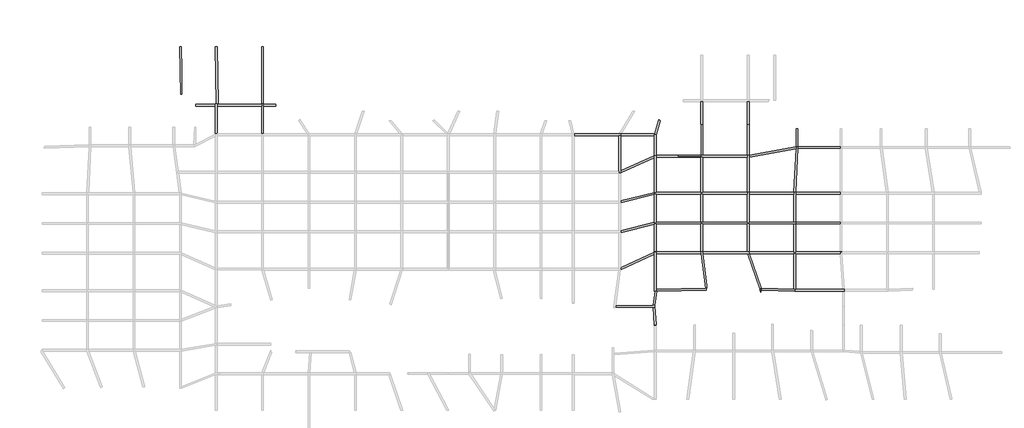
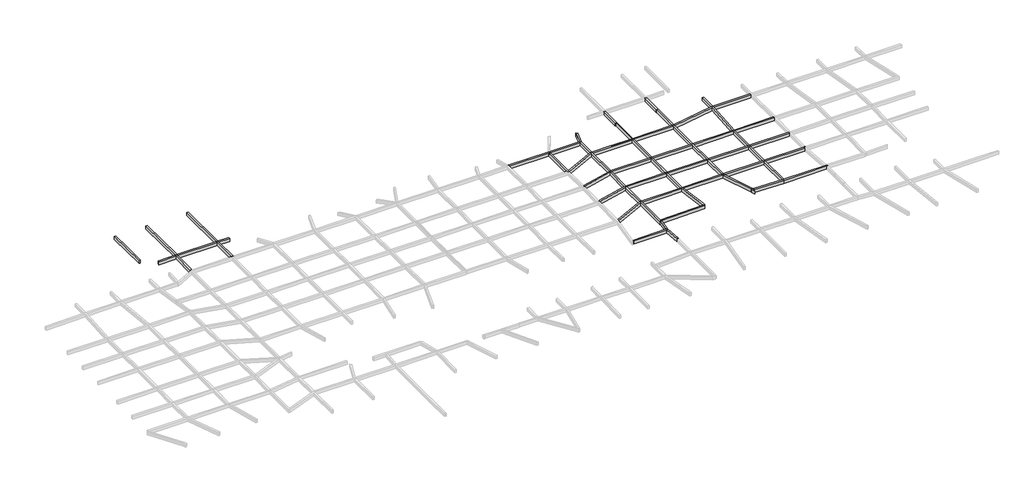
# One storey, part 12 of 15: 57 beams.
"""IFC4 building model written with IfcOpenShell, lengths in millimetres."""

from ifc_helpers import new_model, si_unit, frame, origin, place, context, project, spatial, polyline, outline, extrude, faceted_brep, element, save

model = new_model("IFC4")

# Units and contexts
model_context = context("Model", 3, world=origin())
ifc_project = project(units=[si_unit("LENGTHUNIT", "METRE", prefix="MILLI")], contexts=[model_context])

# Site, building, storey
site = spatial("IfcSite", under=ifc_project)
building = spatial("IfcBuilding", under=site)
storey = spatial("IfcBuildingStorey", under=building, Name="层高", Elevation=3300.0)

# Beams
placement = place(None, origin())
element("IfcBeam", 1, ObjectType="混凝土 - 矩形梁 : KL_beam", at=placement, inside=storey, context=model_context, shape_type="Brep", body=[
    faceted_brep([(161650.3009383, 131842.1448334, 3300.0), (161350.3009383, 131842.1448334, 3300.0), (161350.3009383, 131792.1448334, 3300.0), (161350.3009383, 131492.1448334, 3300.0), (161350.3009383, 126792.1448334, 3300.0), (161650.3009383, 126792.1448334, 3300.0), (161650.3009383, 131492.1448334, 3300.0), (161650.3009383, 131792.1448334, 3300.0), (161650.3009383, 131842.1448334, 2700.0), (161650.3009383, 126792.1448334, 2700.0), (161650.3009383, 131492.1448334, 2700.0), (161650.3009383, 131792.1448334, 2700.0), (161350.3009383, 131842.1448334, 2700.0), (161350.3009383, 126792.1448334, 2700.0), (161350.3009383, 131492.1448334, 2700.0), (161350.3009383, 131792.1448334, 2700.0)], [[[0, 1, 2, 3, 4, 5, 6, 7]], [[8, 0, 7, 6, 5, 9, 10, 11]], [[12, 8, 11, 10, 9, 13, 14, 15]], [[1, 12, 15, 14, 13, 4, 3, 2]], [[5, 4, 13, 9]], [[1, 0, 8, 12]]]),
])
element("IfcBeam", 2, ObjectType="混凝土 - 矩形梁 : KL_beam", at=placement, inside=storey, context=model_context, shape_type="Brep", body=[
    faceted_brep([(221650.3009384, 126492.1448336, 2700.0), (221650.3009384, 126492.1448336, 3300.0), (221350.3009384, 126492.1448336, 3300.0), (213892.2921833, 126492.1448336, 3300.0), (213892.2921833, 126492.1448336, 2700.0), (221350.3009384, 126492.1448336, 2700.0), (213850.3009384, 126792.1448336, 3300.0), (213850.3009384, 126792.1448336, 2700.0), (213850.3009384, 126660.5625177, 2700.0), (213850.3009384, 126660.5625177, 3300.0), (221650.3009384, 126792.1448336, 3300.0), (221414.7215056, 126792.1448336, 3300.0), (221650.3009384, 126792.1448336, 2700.0), (221414.7215056, 126792.1448336, 2700.0)], [[[0, 1, 2, 3, 4, 5]], [[6, 7, 8, 9]], [[1, 10, 11, 6, 9, 3, 2]], [[12, 0, 5, 4, 8, 7, 13]], [[7, 6, 11, 10, 12, 13]], [[4, 3, 9, 8]], [[10, 1, 0, 12]]]),
])
element("IfcBeam", 3, ObjectType="混凝土 - 矩形梁 : KL_beam", at=placement, inside=storey, context=model_context, shape_type="Brep", body=[
    faceted_brep([(221350.3009384, 120192.1448334, 3300.0), (221650.3009384, 120192.1448334, 3300.0), (221650.3009384, 120245.163893, 3300.0), (221650.3009384, 120574.149183, 3300.0), (221650.3009384, 126492.1448336, 3300.0), (221350.3009384, 126492.1448336, 3300.0), (221350.3009384, 120492.1448334, 3300.0), (221650.3009384, 120192.1448334, 2700.0), (221650.3009384, 120245.163893, 2700.0), (221650.3009384, 120574.149183, 2700.0), (221650.3009384, 126492.1448336, 2700.0), (221350.3009384, 120192.1448334, 2700.0), (221350.3009384, 120492.1448334, 2700.0), (221350.3009384, 126492.1448336, 2700.0)], [[[0, 1, 2, 3, 4, 5, 6]], [[1, 7, 8, 9, 10, 4, 3, 2]], [[7, 11, 12, 13, 10, 9, 8]], [[11, 0, 6, 5, 13, 12]], [[5, 4, 10, 13]], [[1, 0, 11, 7]]]),
])
element("IfcBeam", 4, ObjectType="混凝土 - 矩形梁 : KL_beam", at=placement, inside=storey, context=model_context, shape_type="Brep", body=[
    faceted_brep([(227649.8041274, 106937.1819374, 3300.0), (227349.8041274, 106937.1819374, 3300.0), (227349.8041274, 106606.1286193, 3300.0), (227349.8041274, 100394.2440803, 3300.0), (227649.8041274, 100394.2440803, 3300.0), (227649.8041274, 100694.2897788, 3300.0), (227649.8041274, 106691.6486698, 3300.0), (227649.8041274, 106937.1819374, 2700.0), (227649.8041274, 100394.2440803, 2700.0), (227649.8041274, 100694.2897788, 2700.0), (227649.8041274, 106691.6486698, 2700.0), (227349.8041274, 106937.1819374, 2700.0), (227349.8041274, 100394.2440803, 2700.0), (227349.8041274, 106606.1286193, 2700.0)], [[[0, 1, 2, 3, 4, 5, 6]], [[7, 0, 6, 5, 4, 8, 9, 10]], [[11, 7, 10, 9, 8, 12, 13]], [[1, 11, 13, 12, 3, 2]], [[1, 0, 7, 11]], [[3, 12, 8, 4]]]),
])
element("IfcBeam", 5, ObjectType="混凝土 - 矩形梁 : KL_beam", at=placement, inside=storey, context=model_context, shape_type="SweptSolid", body=[
    extrude(outline(polyline([(221650.3009384, 103946.6115658), (221650.3009384, 104032.4006699), (221684.3757671, 104293.5649694), (227349.8041274, 106937.1819374), (227349.8041274, 106606.1286193), (221650.3009384, 103946.6115658)])), frame((0.0, 0.0, 2700.0), z_axis=(0.0, 0.0, 1.0), x_axis=(1.0, 0.0, 0.0)), (0.0, 0.0, 1.0), 600.0),
])
element("IfcBeam", 6, ObjectType="混凝土 - 矩形梁 : KL_beam", at=placement, inside=storey, context=model_context, shape_type="Brep", body=[
    faceted_brep([(227649.8041274, 100694.2897788, 3300.0), (227649.8041274, 100394.2440803, 3300.0), (227761.1939201, 100396.1883964, 3300.0), (236039.6710138, 100540.6897516, 3300.0), (236039.6710138, 100732.444127, 3300.0), (236039.6710138, 100840.73545, 3300.0), (235928.1373023, 100838.7886218, 3300.0), (227349.8041274, 100389.0075609, 3300.0), (227349.8041274, 100389.0075609, 2700.0), (227457.5006433, 100390.8874105, 2700.0), (227649.8041274, 100394.2440803, 2700.0), (227761.1939201, 100396.1883964, 2700.0), (236039.6710138, 100540.6897516, 2700.0), (227457.5006433, 100390.8874105, 3300.0), (227649.8041274, 100694.2897788, 2700.0), (235928.1373023, 100838.7886218, 2700.0), (236039.6710138, 100840.73545, 2700.0), (227349.8041274, 100394.2440803, 3300.0), (227349.8041274, 100394.2440803, 2700.0)], [[[0, 1, 2, 3, 4, 5, 6]], [[7, 8, 9, 10, 11, 12, 3, 2, 1, 13]], [[10, 14, 15, 16, 12, 11]], [[14, 0, 6, 5, 16, 15]], [[8, 7, 17, 18]], [[10, 1, 0, 14]], [[1, 10, 18, 17]], [[17, 7, 13, 1]], [[8, 18, 10, 9]], [[3, 12, 16, 5, 4]]]),
])
element("IfcBeam", 7, ObjectType="混凝土 - 矩形梁 : KL_beam", at=placement, inside=storey, context=model_context, shape_type="Brep", body=[
    faceted_brep([(235431.5832734, 106991.6486698, 3300.0), (235149.8041274, 106991.6486698, 3300.0), (235129.0639103, 106991.6486698, 3300.0), (235168.0249813, 106691.6486698, 3300.0), (235928.1373023, 100838.7886218, 3300.0), (236039.6710138, 100840.73545, 3300.0), (236039.6710138, 100852.444127, 3300.0), (236159.6710138, 100852.444127, 3300.0), (236159.6710138, 101385.3776888, 3300.0), (235470.5443444, 106691.6486698, 3300.0), (235928.1373023, 100838.7886218, 2700.0), (235129.0639103, 106991.6486698, 2700.0), (235168.0249813, 106691.6486698, 2700.0), (235149.8041274, 106991.6486698, 2700.0), (235431.5832734, 106991.6486698, 2700.0), (235470.5443444, 106691.6486698, 2700.0), (236159.6710138, 101385.3776888, 2700.0), (236159.6710138, 100852.444127, 2700.0), (236039.6710138, 100852.444127, 2700.0), (236039.6710138, 100840.73545, 2700.0)], [[[0, 1, 2, 3, 4, 5, 6, 7, 8, 9]], [[10, 4, 3, 2, 11, 12]], [[11, 13, 14, 15, 16, 17, 18, 19, 10, 12]], [[14, 0, 9, 8, 16, 15]], [[4, 10, 19, 5]], [[2, 1, 0, 14, 13, 11]], [[16, 8, 7, 17]], [[6, 18, 17, 7]], [[18, 6, 5, 19]]]),
])
element("IfcBeam", 8, ObjectType="混凝土 - 矩形梁 : KL_beam", at=placement, inside=storey, context=model_context, shape_type="Brep", body=[
    faceted_brep([(227349.8041274, 106991.6486698, 3300.0), (227349.8041274, 106937.1819374, 3300.0), (227649.8041274, 106937.1819374, 3300.0), (227649.8041274, 106746.1154023, 3300.0), (227649.8041274, 106691.6486698, 3300.0), (235168.0249813, 106691.6486698, 3300.0), (235129.0639103, 106991.6486698, 3300.0), (227649.8041274, 106991.6486698, 3300.0), (227649.8041274, 106691.6486698, 2700.0), (235168.0249813, 106691.6486698, 2700.0), (227349.8041274, 106937.1819374, 2700.0), (227349.8041274, 106991.6486698, 2700.0), (227649.8041274, 106991.6486698, 2700.0), (235129.0639103, 106991.6486698, 2700.0), (227649.8041274, 106746.1154023, 2700.0), (227649.8041274, 106937.1819374, 2700.0)], [[[0, 1, 2, 3, 4, 5, 6, 7]], [[4, 8, 9, 5]], [[10, 11, 12, 13, 9, 8, 14, 15]], [[11, 0, 7, 6, 13, 12]], [[0, 11, 10, 1]], [[8, 4, 3, 2, 15, 14]], [[6, 5, 9, 13]], [[15, 2, 1, 10]]]),
])
element("IfcBeam", 9, ObjectType="混凝土 - 矩形梁 : KL_beam", at=placement, inside=storey, context=model_context, shape_type="Brep", body=[
    faceted_brep([(235431.5832734, 106991.6486698, 3300.0), (235470.5443444, 106691.6486698, 3300.0), (242992.8101672, 106691.6486698, 3300.0), (243310.0963715, 106691.6486698, 3300.0), (243249.8041274, 106866.7500612, 3300.0), (243206.7980875, 106991.6486698, 3300.0), (242949.8041274, 106991.6486698, 3300.0), (235449.8041274, 106991.6486698, 3300.0), (235470.5443444, 106691.6486698, 2700.0), (242992.8101672, 106691.6486698, 2700.0), (243310.0963715, 106691.6486698, 2700.0), (235431.5832734, 106991.6486698, 2700.0), (235449.8041274, 106991.6486698, 2700.0), (242949.8041274, 106991.6486698, 2700.0), (243206.7980875, 106991.6486698, 2700.0), (243249.8041274, 106866.7500612, 2700.0)], [[[0, 1, 2, 3, 4, 5, 6, 7]], [[1, 8, 9, 10, 3, 2]], [[8, 11, 12, 13, 14, 15, 10, 9]], [[11, 0, 7, 6, 5, 14, 13, 12]], [[1, 0, 11, 8]], [[5, 4, 3, 10, 15, 14]]]),
])
element("IfcBeam", 10, ObjectType="混凝土 - 矩形梁 : KL_beam", at=placement, inside=storey, context=model_context, shape_type="SweptSolid", body=[
    extrude(outline(polyline([(245239.6710138, 100732.444127), (245239.6710138, 100166.2909583), (245044.7288445, 100732.444127), (245239.6710138, 100732.444127)])), frame((0.0, 0.0, 2700.0), z_axis=(0.0, 0.0, 1.0), x_axis=(1.0, 0.0, 0.0)), (0.0, 0.0, 1.0), 600.0),
    extrude(outline(polyline([(242992.8101672, 106691.6486698), (243310.0963715, 106691.6486698), (245320.6957353, 100852.444127), (245003.4095309, 100852.444127), (242992.8101672, 106691.6486698)])), frame((0.0, 0.0, 2700.0), z_axis=(0.0, 0.0, 1.0), x_axis=(1.0, 0.0, 0.0)), (0.0, 0.0, 1.0), 600.0),
])
element("IfcBeam", 11, ObjectType="混凝土 - 矩形梁 : KL_beam", at=placement, inside=storey, context=model_context, shape_type="Brep", body=[
    faceted_brep([(250897.7707068, 100391.6486698, 3300.0), (250901.8375479, 100691.6486698, 3300.0), (250749.8041274, 100695.7713993, 3300.0), (245359.6710138, 100841.9370275, 3300.0), (245359.6710138, 100541.8267459, 3300.0), (250901.8375479, 100691.6486698, 2700.0), (250749.8041274, 100695.7713993, 2700.0), (245359.6710138, 100841.9370275, 2700.0), (250897.7707068, 100391.6486698, 2700.0), (245359.6710138, 100541.8267459, 2700.0)], [[[0, 1, 2, 3, 4]], [[1, 5, 6, 7, 3, 2]], [[5, 8, 9, 7, 6]], [[8, 0, 4, 9]], [[0, 8, 5, 1]], [[3, 7, 9, 4]]]),
])
element("IfcBeam", 12, ObjectType="混凝土 - 矩形梁 : KL_beam", at=placement, inside=storey, context=model_context, shape_type="Brep", body=[
    faceted_brep([(250901.8375479, 100691.6486698, 3300.0), (250897.7707068, 100391.6486698, 3300.0), (258971.6890495, 100391.6486698, 3300.0), (259271.6890495, 100391.6486698, 3300.0), (259271.6890495, 100546.8867852, 3300.0), (259271.6890495, 100691.6486698, 3300.0), (259261.5663125, 100691.6486698, 3300.0), (258960.833743, 100691.6486698, 3300.0), (251049.8041274, 100691.6486698, 3300.0), (250897.7707068, 100391.6486698, 2700.0), (258971.6890495, 100391.6486698, 2700.0), (259271.6890495, 100391.6486698, 2700.0), (250901.8375479, 100691.6486698, 2700.0), (251049.8041274, 100691.6486698, 2700.0), (258960.833743, 100691.6486698, 2700.0), (259261.5663125, 100691.6486698, 2700.0), (259271.6890495, 100691.6486698, 2700.0), (259271.6890495, 100546.8867852, 2700.0)], [[[0, 1, 2, 3, 4, 5, 6, 7, 8]], [[1, 9, 10, 11, 3, 2]], [[9, 12, 13, 14, 15, 16, 17, 11, 10]], [[12, 0, 8, 7, 6, 5, 16, 15, 14, 13]], [[0, 12, 9, 1]], [[5, 4, 3, 11, 17, 16]]]),
])
element("IfcBeam", 13, ObjectType="混凝土 - 矩形梁 : KL_beam", at=placement, inside=storey, context=model_context, shape_type="Brep", body=[
    faceted_brep([(242949.8041274, 111691.6486698, 3300.0), (243249.8041274, 111691.6486698, 3300.0), (243249.8041274, 111991.6486698, 3300.0), (243249.8041274, 116691.6486698, 3300.0), (243249.8041274, 116991.6486698, 3300.0), (242949.8041274, 116991.6486698, 3300.0), (242949.8041274, 116691.6486698, 3300.0), (242949.8041274, 111991.6486698, 3300.0), (242949.8041274, 111691.6486698, 2700.0), (242949.8041274, 116991.6486698, 2700.0), (242949.8041274, 116691.6486698, 2700.0), (242949.8041274, 111991.6486698, 2700.0), (243249.8041274, 111691.6486698, 2700.0), (243249.8041274, 116991.6486698, 2700.0), (243249.8041274, 116691.6486698, 2700.0), (243249.8041274, 111991.6486698, 2700.0)], [[[0, 1, 2, 3, 4, 5, 6, 7]], [[8, 0, 7, 6, 5, 9, 10, 11]], [[12, 8, 11, 10, 9, 13, 14, 15]], [[1, 12, 15, 14, 13, 4, 3, 2]], [[1, 0, 8, 12]], [[5, 4, 13, 9]]]),
])
element("IfcBeam", 14, ObjectType="混凝土 - 矩形梁 : KL_beam", at=placement, inside=storey, context=model_context, shape_type="Brep", body=[
    faceted_brep([(251049.8041274, 111691.6486698, 3300.0), (251049.8041274, 111991.6486698, 3300.0), (250749.8041274, 111991.6486698, 3300.0), (243249.8041274, 111991.6486698, 3300.0), (243249.8041274, 111691.6486698, 3300.0), (250749.8041274, 111691.6486698, 3300.0), (251049.8041274, 111991.6486698, 2700.0), (250749.8041274, 111991.6486698, 2700.0), (243249.8041274, 111991.6486698, 2700.0), (251049.8041274, 111691.6486698, 2700.0), (250749.8041274, 111691.6486698, 2700.0), (243249.8041274, 111691.6486698, 2700.0)], [[[0, 1, 2, 3, 4, 5]], [[1, 6, 7, 8, 3, 2]], [[6, 9, 10, 11, 8, 7]], [[9, 0, 5, 4, 11, 10]], [[4, 3, 8, 11]], [[1, 0, 9, 6]]]),
])
element("IfcBeam", 15, ObjectType="混凝土 - 矩形梁 : KL_beam", at=placement, inside=storey, context=model_context, shape_type="Brep", body=[
    faceted_brep([(251049.8041274, 116991.6486698, 3300.0), (250757.4594423, 116991.6486698, 3300.0), (250749.8041274, 116991.6486698, 3300.0), (250749.8041274, 116691.6486698, 3300.0), (250749.8041274, 111991.6486698, 3300.0), (251049.8041274, 111991.6486698, 3300.0), (251049.8041274, 116691.6486698, 3300.0), (250749.8041274, 116991.6486698, 2700.0), (250749.8041274, 116691.6486698, 2700.0), (250749.8041274, 111991.6486698, 2700.0), (250757.4594423, 116991.6486698, 2700.0), (251049.8041274, 116991.6486698, 2700.0), (251049.8041274, 116691.6486698, 2700.0), (251049.8041274, 111991.6486698, 2700.0)], [[[0, 1, 2, 3, 4, 5, 6]], [[2, 7, 8, 9, 4, 3]], [[7, 10, 11, 12, 13, 9, 8]], [[11, 0, 6, 5, 13, 12]], [[5, 4, 9, 13]], [[2, 1, 0, 11, 10, 7]]]),
])
element("IfcBeam", 16, ObjectType="混凝土 - 矩形梁 : KL_beam", at=placement, inside=storey, context=model_context, shape_type="SweptSolid", body=[
    extrude(outline(polyline([(243249.8041274, 116691.6486698), (243249.8041274, 116991.6486698), (250749.8041274, 116991.6486698), (250749.8041274, 116691.6486698), (243249.8041274, 116691.6486698)])), frame((0.0, 0.0, 2700.0), z_axis=(0.0, 0.0, 1.0), x_axis=(1.0, 0.0, 0.0)), (0.0, 0.0, 1.0), 600.0),
])
element("IfcBeam", 17, ObjectType="混凝土 - 矩形梁 : KL_beam", at=placement, inside=storey, context=model_context, shape_type="Brep", body=[
    faceted_brep([(235149.8041274, 116991.6486698, 3300.0), (235149.8041274, 116691.6486698, 3300.0), (235449.8041274, 116691.6486698, 3300.0), (242949.8041274, 116691.6486698, 3300.0), (242949.8041274, 116991.6486698, 3300.0), (235449.8041274, 116991.6486698, 3300.0), (235149.8041274, 116691.6486698, 2700.0), (235449.8041274, 116691.6486698, 2700.0), (242949.8041274, 116691.6486698, 2700.0), (235149.8041274, 116991.6486698, 2700.0), (235449.8041274, 116991.6486698, 2700.0), (242949.8041274, 116991.6486698, 2700.0)], [[[0, 1, 2, 3, 4, 5]], [[1, 6, 7, 8, 3, 2]], [[6, 9, 10, 11, 8, 7]], [[9, 0, 5, 4, 11, 10]], [[4, 3, 8, 11]], [[1, 0, 9, 6]]]),
])
element("IfcBeam", 18, ObjectType="混凝土 - 矩形梁 : KL_beam", at=placement, inside=storey, context=model_context, shape_type="Brep", body=[
    faceted_brep([(235149.8041274, 111991.6486698, 3300.0), (235149.8041274, 111691.6486698, 3300.0), (235449.8041274, 111691.6486698, 3300.0), (242949.8041274, 111691.6486698, 3300.0), (242949.8041274, 111991.6486698, 3300.0), (235449.8041274, 111991.6486698, 3300.0), (235149.8041274, 111691.6486698, 2700.0), (235449.8041274, 111691.6486698, 2700.0), (242949.8041274, 111691.6486698, 2700.0), (235149.8041274, 111991.6486698, 2700.0), (235449.8041274, 111991.6486698, 2700.0), (242949.8041274, 111991.6486698, 2700.0)], [[[0, 1, 2, 3, 4, 5]], [[1, 6, 7, 8, 3, 2]], [[6, 9, 10, 11, 8, 7]], [[9, 0, 5, 4, 11, 10]], [[4, 3, 8, 11]], [[1, 0, 9, 6]]]),
])
element("IfcBeam", 19, ObjectType="混凝土 - 矩形梁 : KL_beam", at=placement, inside=storey, context=model_context, shape_type="SweptSolid", body=[
    extrude(outline(polyline([(235149.8041274, 116691.6486698), (235449.8041274, 116691.6486698), (235449.8041274, 111991.6486698), (235149.8041274, 111991.6486698), (235149.8041274, 116691.6486698)])), frame((0.0, 0.0, 2700.0), z_axis=(0.0, 0.0, 1.0), x_axis=(1.0, 0.0, 0.0)), (0.0, 0.0, 1.0), 600.0),
])
element("IfcBeam", 20, ObjectType="混凝土 - 矩形梁 : KL_beam", at=placement, inside=storey, context=model_context, shape_type="Brep", body=[
    faceted_brep([(243249.8041274, 123192.3894162, 3300.0), (242949.8041274, 123192.3894162, 3300.0), (242949.8041274, 122892.3894162, 3300.0), (242949.8041274, 116991.6486698, 3300.0), (243249.8041274, 116991.6486698, 3300.0), (243249.8041274, 122917.161732, 3300.0), (242949.8041274, 123192.3894162, 2700.0), (242949.8041274, 122892.3894162, 2700.0), (242949.8041274, 116991.6486698, 2700.0), (243249.8041274, 123192.3894162, 2700.0), (243249.8041274, 122917.161732, 2700.0), (243249.8041274, 116991.6486698, 2700.0)], [[[0, 1, 2, 3, 4, 5]], [[1, 6, 7, 8, 3, 2]], [[6, 9, 10, 11, 8, 7]], [[9, 0, 5, 4, 11, 10]], [[4, 3, 8, 11]], [[1, 0, 9, 6]]]),
])
element("IfcBeam", 21, ObjectType="混凝土 - 矩形梁 : KL_beam", at=placement, inside=storey, context=model_context, shape_type="Brep", body=[
    faceted_brep([(242949.8041274, 122892.3894162, 3300.0), (242949.8041274, 123192.3894162, 3300.0), (235449.8041274, 123192.3894162, 3300.0), (235209.8041277, 123192.3894162, 3300.0), (235209.8041277, 122892.3894162, 3300.0), (235449.8041274, 122892.3894162, 3300.0), (242949.8041274, 122892.3894162, 2700.0), (235209.8041277, 122892.3894162, 2700.0), (235449.8041274, 122892.3894162, 2700.0), (242949.8041274, 123192.3894162, 2700.0), (235209.8041277, 123192.3894162, 2700.0), (235449.8041274, 123192.3894162, 2700.0)], [[[0, 1, 2, 3, 4, 5]], [[6, 0, 5, 4, 7, 8]], [[9, 6, 8, 7, 10, 11]], [[1, 9, 11, 10, 3, 2]], [[1, 0, 6, 9]], [[4, 3, 10, 7]]]),
])
element("IfcBeam", 22, ObjectType="混凝土 - 矩形梁 : KL_beam", at=placement, inside=storey, context=model_context, shape_type="Brep", body=[
    faceted_brep([(235149.8041274, 116991.6486698, 3300.0), (235449.8041274, 116991.6486698, 3300.0), (235449.8041274, 122892.3894162, 3300.0), (235209.8041277, 122892.3894162, 3300.0), (235149.8041274, 122892.3894162, 3300.0), (235449.8041274, 116991.6486698, 2700.0), (235449.8041274, 122892.3894162, 2700.0), (235149.8041274, 116991.6486698, 2700.0), (235149.8041274, 122892.3894162, 2700.0), (235209.8041277, 122892.3894162, 2700.0)], [[[0, 1, 2, 3, 4]], [[1, 5, 6, 2]], [[5, 7, 8, 9, 6]], [[7, 0, 4, 8]], [[1, 0, 7, 5]], [[4, 3, 2, 6, 9, 8]]]),
])
element("IfcBeam", 23, ObjectType="混凝土 - 矩形梁 : KL_beam", at=placement, inside=storey, context=model_context, shape_type="Brep", body=[
    faceted_brep([(227349.8041274, 116991.6486698, 3300.0), (227349.8041274, 116958.7721753, 3300.0), (227349.8041274, 116691.6486698, 3300.0), (227518.2655284, 116691.6486698, 3300.0), (227649.8041274, 116691.6486698, 3300.0), (235149.8041274, 116691.6486698, 3300.0), (235149.8041274, 116991.6486698, 3300.0), (227649.8041274, 116991.6486698, 3300.0), (227349.8041274, 116691.6486698, 2700.0), (227518.2655284, 116691.6486698, 2700.0), (227649.8041274, 116691.6486698, 2700.0), (235149.8041274, 116691.6486698, 2700.0), (227349.8041274, 116958.7721753, 2700.0), (227349.8041274, 116991.6486698, 2700.0), (227649.8041274, 116991.6486698, 2700.0), (235149.8041274, 116991.6486698, 2700.0)], [[[0, 1, 2, 3, 4, 5, 6, 7]], [[2, 8, 9, 10, 11, 5, 4, 3]], [[8, 12, 13, 14, 15, 11, 10, 9]], [[13, 0, 7, 6, 15, 14]], [[6, 5, 11, 15]], [[2, 1, 0, 13, 12, 8]]]),
])
element("IfcBeam", 24, ObjectType="混凝土 - 矩形梁 : KL_beam", at=placement, inside=storey, context=model_context, shape_type="Brep", body=[
    faceted_brep([(227649.8041274, 123139.3703566, 3300.0), (227349.8041274, 123139.3703566, 3300.0), (227349.8041274, 122810.3850665, 3300.0), (227349.8041274, 116991.6486698, 3300.0), (227649.8041274, 116991.6486698, 3300.0), (227649.8041274, 122892.3894162, 3300.0), (227349.8041274, 123139.3703566, 2700.0), (227349.8041274, 122810.3850665, 2700.0), (227349.8041274, 116991.6486698, 2700.0), (227649.8041274, 123139.3703566, 2700.0), (227649.8041274, 122892.3894162, 2700.0), (227649.8041274, 116991.6486698, 2700.0)], [[[0, 1, 2, 3, 4, 5]], [[1, 6, 7, 8, 3, 2]], [[6, 9, 10, 11, 8, 7]], [[9, 0, 5, 4, 11, 10]], [[4, 3, 8, 11]], [[0, 9, 6, 1]]]),
])
element("IfcBeam", 25, ObjectType="混凝土 - 矩形梁 : KL_beam", at=placement, inside=storey, context=model_context, shape_type="Brep", body=[
    faceted_brep([(227649.8041274, 126621.0726799, 3300.0), (227349.8041274, 126663.2169868, 3300.0), (227349.8041274, 126492.1448336, 3300.0), (227349.8041274, 123139.3703566, 3300.0), (227649.8041274, 123139.3703566, 3300.0), (227649.8041274, 123192.3894162, 3300.0), (227649.8041274, 126621.0726799, 2700.0), (227649.8041274, 123139.3703566, 2700.0), (227649.8041274, 123192.3894162, 2700.0), (227349.8041274, 126663.2169868, 2700.0), (227349.8041274, 123139.3703566, 2700.0), (227349.8041274, 126492.1448336, 2700.0)], [[[0, 1, 2, 3, 4, 5]], [[6, 0, 5, 4, 7, 8]], [[9, 6, 8, 7, 10, 11]], [[1, 9, 11, 10, 3, 2]], [[4, 3, 10, 7]], [[1, 0, 6, 9]]]),
])
element("IfcBeam", 26, ObjectType="混凝土 - 矩形梁 : KL_beam", at=placement, inside=storey, context=model_context, shape_type="Brep", body=[
    faceted_brep([(227349.8041274, 123139.3703566, 3300.0), (221650.3009384, 120574.149183, 3300.0), (221650.3009384, 120492.1448334, 3300.0), (221650.3009384, 120245.163893, 3300.0), (227349.8041274, 122810.3850665, 3300.0), (221650.3009384, 120245.163893, 2700.0), (227349.8041274, 122810.3850665, 2700.0), (221650.3009384, 120574.149183, 2700.0), (227349.8041274, 123139.3703566, 2700.0), (221650.3009384, 120492.1448334, 2700.0)], [[[0, 1, 2, 3, 4]], [[3, 5, 6, 4]], [[7, 8, 6, 5, 9]], [[1, 0, 8, 7]], [[5, 3, 2, 1, 7, 9]], [[0, 4, 6, 8]]]),
])
element("IfcBeam", 27, ObjectType="混凝土 - 矩形梁 : KL_beam", at=placement, inside=storey, context=model_context, shape_type="Brep", body=[
    faceted_brep([(221518.7623395, 115192.1448334, 3300.0), (221350.3009384, 115192.1448334, 3300.0), (221350.3009384, 115150.0399275, 3300.0), (221350.3009384, 115192.1448334, 2700.0), (221518.7623395, 115192.1448334, 2700.0), (221350.3009384, 115150.0399275, 2700.0)], [[[0, 1, 2]], [[3, 4, 5]], [[2, 5, 4, 0]], [[5, 2, 1, 3]], [[1, 0, 4, 3]]]),
    faceted_brep([(221650.3009384, 115534.2497393, 2700.0), (221650.3009384, 115534.2497393, 3300.0), (227349.8041274, 116958.7721753, 3300.0), (227349.8041274, 116958.7721753, 2700.0), (221650.3009384, 115492.1448334, 2700.0), (221650.3009384, 115225.0213279, 2700.0), (221650.3009384, 115225.0213279, 3300.0), (221650.3009384, 115492.1448334, 3300.0), (227349.8041274, 116691.6486698, 2700.0), (227349.8041274, 116691.6486698, 3300.0), (227518.2655284, 116691.6486698, 3300.0), (227518.2655284, 116691.6486698, 2700.0), (227349.8041274, 116649.5437639, 3300.0), (227349.8041274, 116649.5437639, 2700.0)], [[[0, 1, 2, 3]], [[1, 0, 4, 5, 6, 7]], [[8, 9, 10, 11]], [[9, 8, 3, 2]], [[6, 12, 10, 9, 2, 1, 7]], [[0, 3, 8, 11, 13, 5, 4]], [[6, 5, 13, 11, 10, 12]]]),
])
element("IfcBeam", 28, ObjectType="混凝土 - 矩形梁 : KL_beam", at=placement, inside=storey, context=model_context, shape_type="Brep", body=[
    faceted_brep([(227349.8041274, 111691.6486698, 3300.0), (227518.2655284, 111691.6486698, 3300.0), (227649.8041274, 111691.6486698, 3300.0), (227649.8041274, 111991.6486698, 3300.0), (227649.8041274, 116691.6486698, 3300.0), (227518.2655284, 116691.6486698, 3300.0), (227349.8041274, 116649.5437639, 3300.0), (227349.8041274, 111958.7721753, 3300.0), (227649.8041274, 116691.6486698, 2700.0), (227649.8041274, 111691.6486698, 2700.0), (227649.8041274, 111991.6486698, 2700.0), (227518.2655284, 111691.6486698, 2700.0), (227349.8041274, 111691.6486698, 2700.0), (227349.8041274, 111958.7721753, 2700.0), (227349.8041274, 116649.5437639, 2700.0), (227518.2655284, 116691.6486698, 2700.0)], [[[0, 1, 2, 3, 4, 5, 6, 7]], [[8, 4, 3, 2, 9, 10]], [[9, 11, 12, 13, 14, 15, 8, 10]], [[12, 0, 7, 6, 14, 13]], [[4, 8, 15, 5]], [[6, 5, 15, 14]], [[2, 1, 0, 12, 11, 9]]]),
])
element("IfcBeam", 29, ObjectType="混凝土 - 矩形梁 : KL_beam", at=placement, inside=storey, context=model_context, shape_type="SweptSolid", body=[
    extrude(outline(polyline([(235149.8041274, 111991.6486698), (235149.8041274, 111691.6486698), (227649.8041274, 111691.6486698), (227649.8041274, 111991.6486698), (235149.8041274, 111991.6486698)])), frame((0.0, 0.0, 2700.0), z_axis=(0.0, 0.0, 1.0), x_axis=(1.0, 0.0, 0.0)), (0.0, 0.0, 1.0), 600.0),
])
element("IfcBeam", 30, ObjectType="混凝土 - 矩形梁 : KL_beam", at=placement, inside=storey, context=model_context, shape_type="Brep", body=[
    faceted_brep([(221481.8395373, 110492.1448334, 3300.0), (221650.3009384, 110492.1448334, 3300.0), (221650.3009384, 110225.0213279, 3300.0), (227349.8041274, 111649.5437639, 3300.0), (227518.2655284, 111691.6486698, 3300.0), (227349.8041274, 111691.6486698, 3300.0), (227349.8041274, 111958.7721753, 3300.0), (221650.3009384, 110534.2497393, 3300.0), (221650.3009384, 110225.0213279, 2700.0), (227349.8041274, 111649.5437639, 2700.0), (227518.2655284, 111691.6486698, 2700.0), (221650.3009384, 110492.1448334, 2700.0), (221481.8395373, 110492.1448334, 2700.0), (221650.3009384, 110534.2497393, 2700.0), (227349.8041274, 111958.7721753, 2700.0), (227349.8041274, 111691.6486698, 2700.0)], [[[0, 1, 2, 3, 4, 5, 6, 7]], [[2, 8, 9, 10, 4, 3]], [[11, 12, 13, 14, 15, 10, 9, 8]], [[12, 0, 7, 6, 14, 13]], [[11, 1, 0, 12]], [[1, 11, 8, 2]], [[5, 15, 14, 6]], [[15, 5, 4, 10]]]),
])
element("IfcBeam", 31, ObjectType="混凝土 - 矩形梁 : KL_beam", at=placement, inside=storey, context=model_context, shape_type="SweptSolid", body=[
    extrude(outline(polyline([(227649.8041274, 106991.6486698), (227349.8041274, 106991.6486698), (227349.8041274, 111649.5437639), (227518.2655284, 111691.6486698), (227649.8041274, 111691.6486698), (227649.8041274, 106991.6486698)])), frame((0.0, 0.0, 2700.0), z_axis=(0.0, 0.0, 1.0), x_axis=(1.0, 0.0, 0.0)), (0.0, 0.0, 1.0), 600.0),
])
element("IfcBeam", 32, ObjectType="混凝土 - 矩形梁 : KL_beam", at=placement, inside=storey, context=model_context, shape_type="Brep", body=[
    faceted_brep([(235149.8041274, 106991.6486698, 3300.0), (235431.5832734, 106991.6486698, 3300.0), (235449.8041274, 106991.6486698, 3300.0), (235449.8041274, 111691.6486698, 3300.0), (235149.8041274, 111691.6486698, 3300.0), (235149.8041274, 106991.6486698, 2700.0), (235149.8041274, 111691.6486698, 2700.0), (235449.8041274, 106991.6486698, 2700.0), (235431.5832734, 106991.6486698, 2700.0), (235449.8041274, 111691.6486698, 2700.0)], [[[0, 1, 2, 3, 4]], [[5, 0, 4, 6]], [[7, 8, 5, 6, 9]], [[2, 7, 9, 3]], [[0, 5, 8, 7, 2, 1]], [[4, 3, 9, 6]]]),
])
element("IfcBeam", 33, ObjectType="混凝土 - 矩形梁 : KL_beam", at=placement, inside=storey, context=model_context, shape_type="Brep", body=[
    faceted_brep([(153550.3009381, 131842.1448334, 3300.0), (153850.3009381, 131842.1448334, 3300.0), (153850.3009381, 131842.1448334, 2700.0), (153550.3009381, 131842.1448334, 2700.0), (153550.3009381, 131792.1448334, 3300.0), (153550.3009381, 131492.1448334, 3300.0), (153550.3009381, 126792.1448334, 3300.0), (153664.2891243, 126792.1448334, 3300.0), (153850.3009381, 126886.9225864, 3300.0), (153850.3009381, 131492.1448334, 3300.0), (153850.3009381, 131792.1448334, 3300.0), (153850.3009381, 126886.9225864, 2700.0), (153850.3009381, 131492.1448334, 2700.0), (153850.3009381, 131792.1448334, 2700.0), (153664.2891243, 126792.1448334, 2700.0), (153550.3009381, 126792.1448334, 2700.0), (153550.3009381, 131492.1448334, 2700.0), (153550.3009381, 131792.1448334, 2700.0)], [[[0, 1, 2, 3]], [[1, 0, 4, 5, 6, 7, 8, 9, 10]], [[2, 1, 10, 9, 8, 11, 12, 13]], [[3, 2, 13, 12, 11, 14, 15, 16, 17]], [[0, 3, 17, 16, 15, 6, 5, 4]], [[6, 15, 14, 7]], [[8, 7, 14, 11]]]),
])
element("IfcBeam", 34, ObjectType="混凝土 - 矩形梁 : KL_beam", at=placement, inside=storey, context=model_context, shape_type="SweptSolid", body=[
    extrude(outline(polyline([(147851.515391, 141482.6292767), (147933.8101639, 137619.2886034), (147933.8101639, 133452.6274413), (147722.4980492, 133452.6274413), (147551.4473359, 141482.6292767), (147851.515391, 141482.6292767)])), frame((0.0, 0.0, 2700.0), z_axis=(0.0, 0.0, 1.0), x_axis=(1.0, 0.0, 0.0)), (0.0, 0.0, 1.0), 600.0),
])
element("IfcBeam", 35, ObjectType="混凝土 - 矩形梁 : KL_beam", at=placement, inside=storey, context=model_context, shape_type="SweptSolid", body=[
    extrude(outline(polyline([(161650.3009383, 131842.1448334), (161350.3009383, 131842.1448334), (161350.3009383, 141482.6292767), (161650.3009383, 141482.6292767), (161650.3009383, 131842.1448334)])), frame((0.0, 0.0, 2700.0), z_axis=(0.0, 0.0, 1.0), x_axis=(1.0, 0.0, 0.0)), (0.0, 0.0, 1.0), 600.0),
])
element("IfcBeam", 36, ObjectType="混凝土 - 矩形梁 : KL_beam", at=placement, inside=storey, context=model_context, shape_type="SweptSolid", body=[
    extrude(outline(polyline([(154026.5791632, 131845.2436707), (153726.6248547, 131840.0079487), (153558.3122733, 141482.6292767), (153858.3579717, 141482.6292767), (154026.5791632, 131845.2436707)])), frame((0.0, 0.0, 2700.0), z_axis=(0.0, 0.0, 1.0), x_axis=(1.0, 0.0, 0.0)), (0.0, 0.0, 1.0), 600.0),
])
element("IfcBeam", 37, ObjectType="混凝土 - 矩形梁 : KL_beam", at=placement, inside=storey, context=model_context, shape_type="Brep", body=[
    faceted_brep([(242949.8041274, 123192.3894162, 3300.0), (243249.8041274, 123192.3894162, 3300.0), (243249.8041274, 123222.062147, 3300.0), (243249.8041274, 128327.7400891, 3300.0), (242949.8041274, 128327.7400891, 3300.0), (242949.8041274, 123192.3894162, 2700.0), (242949.8041274, 128327.7400891, 2700.0), (243249.8041274, 123192.3894162, 2700.0), (243249.8041274, 128327.7400891, 2700.0), (243249.8041274, 123222.062147, 2700.0)], [[[0, 1, 2, 3, 4]], [[5, 0, 4, 6]], [[7, 5, 6, 8, 9]], [[1, 7, 9, 8, 3, 2]], [[1, 0, 5, 7]], [[4, 3, 8, 6]]]),
    faceted_brep([(242949.8041274, 132239.648667, 3300.0), (243249.8041274, 132239.648667, 3300.0), (243249.8041274, 132239.648667, 2700.0), (242949.8041274, 132239.648667, 2700.0), (243249.8041274, 128447.7400891, 3300.0), (242949.8041274, 128447.7400891, 3300.0), (242949.8041274, 128447.7400891, 2700.0), (243249.8041274, 128447.7400891, 2700.0)], [[[0, 1, 2, 3]], [[4, 5, 6, 7]], [[1, 0, 5, 4]], [[0, 3, 6, 5]], [[3, 2, 7, 6]], [[2, 1, 4, 7]]]),
])
element("IfcBeam", 38, ObjectType="混凝土 - 矩形梁 : KL_beam", at=placement, inside=storey, context=model_context, shape_type="SweptSolid", body=[
    extrude(outline(polyline([(235449.8041274, 128327.7400891), (235449.8041274, 123192.3894162), (235209.8041277, 123192.3894162), (235209.8041277, 128327.7400891), (235449.8041274, 128327.7400891)])), frame((0.0, 0.0, 2700.0), z_axis=(0.0, 0.0, 1.0), x_axis=(1.0, 0.0, 0.0)), (0.0, 0.0, 1.0), 600.0),
    extrude(outline(polyline([(235149.8041274, 132239.648667), (235449.8041274, 132239.648667), (235449.8041274, 128447.7400891), (235149.8041274, 128447.7400891), (235149.8041274, 132239.648667)])), frame((0.0, 0.0, 2700.0), z_axis=(0.0, 0.0, 1.0), x_axis=(1.0, 0.0, 0.0)), (0.0, 0.0, 1.0), 600.0),
])
element("IfcBeam", 39, ObjectType="混凝土 - 矩形梁 : KL_beam", at=placement, inside=storey, context=model_context, shape_type="Brep", body=[
    faceted_brep([(227649.8041274, 123192.3894162, 3300.0), (227649.8041274, 123139.3703566, 3300.0), (227649.8041274, 122892.3894162, 3300.0), (235089.8041277, 122892.3894162, 3300.0), (235089.8041277, 122931.6486698, 3300.0), (231369.8041277, 122931.6486698, 3300.0), (231249.8041277, 122931.6486698, 3300.0), (231249.8041277, 123192.3894162, 3300.0), (227649.8041274, 122892.3894162, 2700.0), (235089.8041277, 122892.3894162, 2700.0), (227649.8041274, 123139.3703566, 2700.0), (227649.8041274, 123192.3894162, 2700.0), (231249.8041277, 123192.3894162, 2700.0), (231249.8041277, 122931.6486698, 2700.0), (235089.8041277, 122931.6486698, 2700.0)], [[[0, 1, 2, 3, 4, 5, 6, 7]], [[2, 8, 9, 3]], [[8, 10, 11, 12, 13, 14, 9]], [[11, 0, 7, 12]], [[8, 2, 1, 0, 11, 10]], [[4, 14, 13, 6, 5]], [[3, 9, 14, 4]], [[6, 13, 12, 7]]]),
    faceted_brep([(235089.8041277, 123192.3894162, 2700.0), (235089.8041277, 123192.3894162, 3300.0), (235089.8041277, 123051.6486698, 3300.0), (235089.8041277, 123051.6486698, 2700.0), (231369.8041277, 123051.6486698, 3300.0), (231369.8041277, 123051.6486698, 2700.0), (231369.8041277, 123192.3894162, 3300.0), (231369.8041277, 123192.3894162, 2700.0)], [[[0, 1, 2, 3]], [[2, 4, 5, 3]], [[4, 6, 7, 5]], [[2, 1, 6, 4]], [[0, 3, 5, 7]], [[1, 0, 7, 6]]]),
])
element("IfcBeam", 40, ObjectType="混凝土 - 矩形梁 : KL_beam", at=placement, inside=storey, context=model_context, shape_type="Brep", body=[
    faceted_brep([(228061.8544031, 129147.5312684, 3300.0), (227386.7572253, 126792.1448336, 3300.0), (227349.8041274, 126663.2169868, 3300.0), (227649.8041274, 126621.0726799, 3300.0), (228339.539526, 129027.5312684, 3300.0), (228140.6969646, 129027.5312684, 3300.0), (228140.6969646, 129147.5312684, 3300.0), (227649.8041274, 126621.0726799, 2700.0), (228339.539526, 129027.5312684, 2700.0), (227349.8041274, 126663.2169868, 2700.0), (227386.7572253, 126792.1448336, 2700.0), (228061.8544031, 129147.5312684, 2700.0), (228140.6969646, 129147.5312684, 2700.0), (228140.6969646, 129027.5312684, 2700.0)], [[[0, 1, 2, 3, 4, 5, 6]], [[3, 7, 8, 4]], [[9, 10, 11, 12, 13, 8, 7]], [[2, 1, 0, 11, 10, 9]], [[11, 0, 6, 12]], [[2, 9, 7, 3]], [[13, 5, 4, 8]], [[5, 13, 12, 6]]]),
])
element("IfcBeam", 41, ObjectType="混凝土 - 矩形梁 : KL_beam", at=placement, inside=storey, context=model_context, shape_type="Brep", body=[
    faceted_brep([(221650.3009384, 126792.1448336, 3300.0), (221650.3009384, 126492.1448336, 3300.0), (227349.8041274, 126492.1448336, 3300.0), (227349.8041274, 126663.2169868, 3300.0), (227386.7572253, 126792.1448336, 3300.0), (221763.2145762, 126792.1448336, 3300.0), (221650.3009384, 126492.1448336, 2700.0), (227349.8041274, 126492.1448336, 2700.0), (221650.3009384, 126792.1448336, 2700.0), (221763.2145762, 126792.1448336, 2700.0), (227386.7572253, 126792.1448336, 2700.0), (227349.8041274, 126663.2169868, 2700.0)], [[[0, 1, 2, 3, 4, 5]], [[1, 6, 7, 2]], [[6, 8, 9, 10, 11, 7]], [[8, 0, 5, 4, 10, 9]], [[1, 0, 8, 6]], [[3, 2, 7, 11]], [[4, 3, 11, 10]]]),
])
element("IfcBeam", 42, ObjectType="混凝土 - 矩形梁 : KL_beam", at=placement, inside=storey, context=model_context, shape_type="Brep", body=[
    faceted_brep([(250749.8041274, 106691.6486698, 3300.0), (251049.8041274, 106691.6486698, 3300.0), (251049.8041274, 106991.6486698, 3300.0), (251049.8041274, 111691.6486698, 3300.0), (250749.8041274, 111691.6486698, 3300.0), (250749.8041274, 106991.6486698, 3300.0), (251049.8041274, 106691.6486698, 2700.0), (251049.8041274, 106991.6486698, 2700.0), (251049.8041274, 111691.6486698, 2700.0), (250749.8041274, 106691.6486698, 2700.0), (250749.8041274, 106991.6486698, 2700.0), (250749.8041274, 111691.6486698, 2700.0)], [[[0, 1, 2, 3, 4, 5]], [[1, 6, 7, 8, 3, 2]], [[6, 9, 10, 11, 8, 7]], [[9, 0, 5, 4, 11, 10]], [[4, 3, 8, 11]], [[1, 0, 9, 6]]]),
])
element("IfcBeam", 43, ObjectType="混凝土 - 矩形梁 : KL_beam", at=placement, inside=storey, context=model_context, shape_type="Brep", body=[
    faceted_brep([(242949.8041274, 106991.6486698, 3300.0), (243206.7980875, 106991.6486698, 3300.0), (243249.8041274, 106866.7500612, 3300.0), (243249.8041274, 106991.6486698, 3300.0), (243249.8041274, 111691.6486698, 3300.0), (242949.8041274, 111691.6486698, 3300.0), (242949.8041274, 106991.6486698, 2700.0), (242949.8041274, 111691.6486698, 2700.0), (243206.7980875, 106991.6486698, 2700.0), (243249.8041274, 111691.6486698, 2700.0), (243249.8041274, 106991.6486698, 2700.0), (243249.8041274, 106866.7500612, 2700.0)], [[[0, 1, 2, 3, 4, 5]], [[6, 0, 5, 7]], [[8, 6, 7, 9, 10, 11]], [[2, 11, 10, 9, 4, 3]], [[8, 1, 0, 6]], [[1, 8, 11, 2]], [[5, 4, 9, 7]]]),
])
element("IfcBeam", 44, ObjectType="混凝土 - 矩形梁 : KL_beam", at=placement, inside=storey, context=model_context, shape_type="SweptSolid", body=[
    extrude(outline(polyline([(243310.0963715, 106691.6486698), (243249.8041274, 106866.7500612), (243249.8041274, 106991.6486698), (250749.8041274, 106991.6486698), (250749.8041274, 106691.6486698), (243310.0963715, 106691.6486698)])), frame((0.0, 0.0, 2700.0), z_axis=(0.0, 0.0, 1.0), x_axis=(1.0, 0.0, 0.0)), (0.0, 0.0, 1.0), 600.0),
])
element("IfcBeam", 45, ObjectType="混凝土 - 矩形梁 : KL_beam", at=placement, inside=storey, context=model_context, shape_type="SweptSolid", body=[
    extrude(outline(polyline([(250901.8375479, 100691.6486698), (250749.8041274, 100695.7713993), (250749.8041274, 106691.6486698), (251049.8041274, 106691.6486698), (251049.8041274, 100691.6486698), (250901.8375479, 100691.6486698)])), frame((0.0, 0.0, 2700.0), z_axis=(0.0, 0.0, 1.0), x_axis=(1.0, 0.0, 0.0)), (0.0, 0.0, 1.0), 600.0),
])
element("IfcBeam", 46, ObjectType="混凝土 - 矩形梁 : KL_beam", at=placement, inside=storey, context=model_context, shape_type="Brep", body=[
    faceted_brep([(258541.2728714, 106691.6486698, 2700.0), (258541.2728714, 106691.6486698, 3300.0), (251049.8041274, 106691.6486698, 3300.0), (251049.8041274, 106691.6486698, 2700.0), (258821.0273972, 106991.6486698, 3300.0), (258821.0273972, 106991.6486698, 2700.0), (258531.1501343, 106991.6486698, 2700.0), (251049.8041274, 106991.6486698, 2700.0), (251049.8041274, 106991.6486698, 3300.0), (258531.1501343, 106991.6486698, 3300.0), (258521.7581821, 106970.7217277, 2700.0), (258521.7581821, 106970.7217277, 3300.0)], [[[0, 1, 2, 3]], [[4, 5, 6, 7, 8, 9]], [[10, 11, 1, 0]], [[11, 10, 5, 4]], [[3, 2, 8, 7]], [[1, 11, 4, 9, 8, 2]], [[10, 0, 3, 7, 6, 5]]]),
])
element("IfcBeam", 47, ObjectType="混凝土 - 矩形梁 : KL_beam", at=placement, inside=storey, context=model_context, shape_type="SweptSolid", body=[
    extrude(outline(polyline([(251049.8041274, 111691.6486698), (251049.8041274, 111991.6486698), (258531.1501343, 111991.6486698), (258531.1501343, 111691.6486698), (251049.8041274, 111691.6486698)])), frame((0.0, 0.0, 2700.0), z_axis=(0.0, 0.0, 1.0), x_axis=(1.0, 0.0, 0.0)), (0.0, 0.0, 1.0), 600.0),
])
element("IfcBeam", 48, ObjectType="混凝土 - 矩形梁 : KL_beam", at=placement, inside=storey, context=model_context, shape_type="Brep", body=[
    faceted_brep([(251049.8041274, 116991.6486698, 3300.0), (251049.8041274, 116691.6486698, 3300.0), (258549.8041274, 116691.6486698, 3300.0), (258549.8041274, 116991.6486698, 3300.0), (251057.8711461, 116991.6486698, 3300.0), (251049.8041274, 116991.6486698, 2700.0), (258549.8041274, 116991.6486698, 2700.0), (251057.8711461, 116991.6486698, 2700.0), (251049.8041274, 116691.6486698, 2700.0), (258549.8041274, 116691.6486698, 2700.0)], [[[0, 1, 2, 3, 4]], [[5, 0, 4, 3, 6, 7]], [[8, 5, 7, 6, 9]], [[1, 8, 9, 2]], [[1, 0, 5, 8]], [[3, 2, 9, 6]]]),
])
element("IfcBeam", 49, ObjectType="混凝土 - 矩形梁 : KL_beam", at=placement, inside=storey, context=model_context, shape_type="Brep", body=[
    faceted_brep([(251159.2090868, 124657.4885502, 3300.0), (251143.0764937, 124349.6603359, 3300.0), (250757.4594423, 116991.6486698, 3300.0), (251049.8041274, 116991.6486698, 3300.0), (251057.8711461, 116991.6486698, 3300.0), (251445.1356754, 124381.0960874, 3300.0), (251458.7979472, 124641.7877633, 3300.0), (251458.7979472, 124641.7877633, 2700.0), (251057.8711461, 116991.6486698, 2700.0), (251445.1356754, 124381.0960874, 2700.0), (251049.8041274, 116991.6486698, 2700.0), (250757.4594423, 116991.6486698, 2700.0), (251143.0764937, 124349.6603359, 2700.0), (251159.2090868, 124657.4885502, 2700.0)], [[[0, 1, 2, 3, 4, 5, 6]], [[7, 6, 5, 4, 8, 9]], [[8, 10, 11, 12, 13, 7, 9]], [[2, 1, 0, 13, 12, 11]], [[2, 11, 10, 8, 4, 3]], [[0, 6, 7, 13]]]),
])
element("IfcBeam", 50, ObjectType="混凝土 - 矩形梁 : KL_beam", at=placement, inside=storey, context=model_context, shape_type="Brep", body=[
    faceted_brep([(251159.2090868, 124657.4885502, 3300.0), (251152.7909904, 124656.3237717, 3300.0), (243249.8041274, 123222.062147, 3300.0), (243249.8041274, 123192.3894162, 3300.0), (243249.8041274, 122917.161732, 3300.0), (251143.0764937, 124349.6603359, 3300.0), (243249.8041274, 122917.161732, 2700.0), (251143.0764937, 124349.6603359, 2700.0), (243249.8041274, 123222.062147, 2700.0), (251152.7909904, 124656.3237717, 2700.0), (251159.2090868, 124657.4885502, 2700.0), (243249.8041274, 123192.3894162, 2700.0)], [[[0, 1, 2, 3, 4, 5]], [[4, 6, 7, 5]], [[8, 9, 10, 7, 6, 11]], [[2, 1, 0, 10, 9, 8]], [[6, 4, 3, 2, 8, 11]], [[0, 5, 7, 10]]]),
])
element("IfcBeam", 51, ObjectType="混凝土 - 矩形梁 : KL_beam", at=placement, inside=storey, context=model_context, shape_type="Brep", body=[
    faceted_brep([(251159.2090868, 124657.4885502, 3300.0), (251458.7979472, 124641.7877633, 3300.0), (251446.372894, 124404.7036246, 3300.0), (251445.1356754, 124381.0960874, 3300.0), (258549.8041274, 124381.0960874, 3300.0), (258549.8041274, 124681.0960874, 3300.0), (251452.7909904, 124681.0960874, 3300.0), (251160.4463054, 124681.0960874, 3300.0), (251445.1356754, 124381.0960874, 2700.0), (258549.8041274, 124381.0960874, 2700.0), (251458.7979472, 124641.7877633, 2700.0), (251159.2090868, 124657.4885502, 2700.0), (251160.4463054, 124681.0960874, 2700.0), (251452.7909904, 124681.0960874, 2700.0), (258549.8041274, 124681.0960874, 2700.0), (251446.372894, 124404.7036246, 2700.0)], [[[0, 1, 2, 3, 4, 5, 6, 7]], [[3, 8, 9, 4]], [[10, 11, 12, 13, 14, 9, 8, 15]], [[12, 7, 6, 5, 14, 13]], [[11, 0, 7, 12]], [[1, 10, 15, 8, 3, 2]], [[10, 1, 0, 11]], [[5, 4, 9, 14]]]),
])
element("IfcBeam", 52, ObjectType="混凝土 - 矩形梁 : KL_beam", at=placement, inside=storey, context=model_context, shape_type="SweptSolid", body=[
    extrude(outline(polyline([(251159.2090868, 124657.4885502), (251152.7909904, 124656.3237717), (251152.7909904, 127629.6486698), (251452.7909904, 127629.6486698), (251452.7909904, 124681.0960874), (251160.4463054, 124681.0960874), (251159.2090868, 124657.4885502)])), frame((0.0, 0.0, 2700.0), z_axis=(0.0, 0.0, 1.0), x_axis=(1.0, 0.0, 0.0)), (0.0, 0.0, 1.0), 600.0),
])
element("IfcBeam", 53, ObjectType="混凝土 - 矩形梁 : KL_beam", at=placement, inside=storey, context=model_context, shape_type="Brep", body=[
    faceted_brep([(227383.5570279, 97709.162288, 3300.0), (227403.5809389, 97851.6398179, 3300.0), (227425.8294013, 98009.9458535, 3300.0), (227122.1361245, 98004.6448676, 3300.0), (220849.5577256, 97895.1566044, 3300.0), (220810.3205741, 97594.426019, 3300.0), (227113.141432, 97704.4421663, 3300.0), (227383.5570279, 97709.162288, 2700.0), (220810.3205741, 97594.426019, 2700.0), (227113.141432, 97704.4421663, 2700.0), (227425.8294013, 98009.9458535, 2700.0), (227403.5809389, 97851.6398179, 2700.0), (220849.5577256, 97895.1566044, 2700.0), (227122.1361245, 98004.6448676, 2700.0)], [[[0, 1, 2, 3, 4, 5, 6]], [[7, 0, 6, 5, 8, 9]], [[10, 11, 7, 9, 8, 12, 13]], [[2, 10, 13, 12, 4, 3]], [[5, 4, 12, 8]], [[2, 1, 0, 7, 11, 10]]]),
])
element("IfcBeam", 54, ObjectType="混凝土 - 矩形梁 : KL_beam", at=placement, inside=storey, context=model_context, shape_type="Brep", body=[
    faceted_brep([(227122.1361245, 98004.6448676, 3300.0), (227425.8294013, 98009.9458535, 3300.0), (227761.1939201, 100396.1883964, 3300.0), (227649.8041274, 100394.2440803, 3300.0), (227457.5006433, 100390.8874105, 3300.0), (227122.1361245, 98004.6448676, 2700.0), (227457.5006433, 100390.8874105, 2700.0), (227425.8294013, 98009.9458535, 2700.0), (227649.8041274, 100394.2440803, 2700.0), (227761.1939201, 100396.1883964, 2700.0)], [[[0, 1, 2, 3, 4]], [[5, 0, 4, 6]], [[7, 5, 6, 8, 9]], [[1, 7, 9, 2]], [[1, 0, 5, 7]], [[4, 3, 2, 9, 8, 6]]]),
])
element("IfcBeam", 55, ObjectType="混凝土 - 矩形梁 : KL_beam", at=placement, inside=storey, context=model_context, shape_type="SweptSolid", body=[
    extrude(outline(polyline([(227629.4690157, 94621.2898205), (227329.4690157, 94610.8135896), (227328.1494068, 94629.6848758), (227628.8819762, 94629.6848758), (227629.4690157, 94621.2898205)])), frame((0.0, 0.0, 2700.0), z_axis=(0.0, 0.0, 1.0), x_axis=(1.0, 0.0, 0.0)), (0.0, 0.0, 1.0), 600.0),
    extrude(outline(polyline([(227113.141432, 97704.4421663), (227383.5570279, 97709.162288), (227403.5809389, 97851.6398179), (227620.4907588, 94749.6848758), (227319.7581894, 94749.6848758), (227113.141432, 97704.4421663)])), frame((0.0, 0.0, 2700.0), z_axis=(0.0, 0.0, 1.0), x_axis=(1.0, 0.0, 0.0)), (0.0, 0.0, 1.0), 600.0),
])
element("IfcBeam", 56, ObjectType="混凝土 - 矩形梁 : KL_beam", at=placement, inside=storey, context=model_context, shape_type="SweptSolid", body=[
    extrude(outline(polyline([(161350.3009383, 131792.1448334), (161350.3009383, 131492.1448334), (153850.3009381, 131492.1448334), (153850.3009381, 131792.1448334), (161350.3009383, 131792.1448334)])), frame((0.0, 0.0, 2700.0), z_axis=(0.0, 0.0, 1.0), x_axis=(1.0, 0.0, 0.0)), (0.0, 0.0, 1.0), 600.0),
    extrude(outline(polyline([(150309.8101643, 131492.1448334), (150309.8101643, 131792.1448334), (153550.3009381, 131792.1448334), (153550.3009381, 131492.1448334), (150309.8101643, 131492.1448334)])), frame((0.0, 0.0, 2700.0), z_axis=(0.0, 0.0, 1.0), x_axis=(1.0, 0.0, 0.0)), (0.0, 0.0, 1.0), 600.0),
])
element("IfcBeam", 57, ObjectType="混凝土 - 矩形梁 : KL_beam", at=placement, inside=storey, context=model_context, shape_type="SweptSolid", body=[
    extrude(outline(polyline([(163740.6969648, 131792.1448334), (163740.6969648, 131492.1448334), (161650.3009383, 131492.1448334), (161650.3009383, 131792.1448334), (163740.6969648, 131792.1448334)])), frame((0.0, 0.0, 2700.0), z_axis=(0.0, 0.0, 1.0), x_axis=(1.0, 0.0, 0.0)), (0.0, 0.0, 1.0), 600.0),
])

save(model, "model.ifc")

# Revit data of these elements
# Type "混凝土 - 矩形梁 : KL_beam"
#   Length [instance default] = 1524 mm
#   b = 300 mm
#   h = 600 mm
#   Structural Material [instance default] = 混凝土 - 现场浇注混凝土
#   Assembly Code = ""
# Elements 1, 2, 3, 4, 5, 6, 7, 8, 9, 10, 11, 12, 13, 14, 15, 16, 17, 18, 19, 20, 21, 22, 23, 24, 25, 26, 27, 28, 29, 30, 31, 32, 33, 34, 35, 36, 37, 38, 39, 40, 41, 42, 43, 44, 45, 46, 47, 48, 49, 50, 51, 52, 53, 54, 55, 56, 57 (IfcBeam, "混凝土 - 矩形梁 : KL_beam")
#   Comments = ""
#   Structural Material = none
#   Phase Created = 新构造
# Materials
#   "混凝土 - 现场浇注混凝土": class "混凝土", colour RGB 192 192 192, transparency 0
